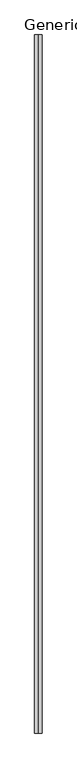
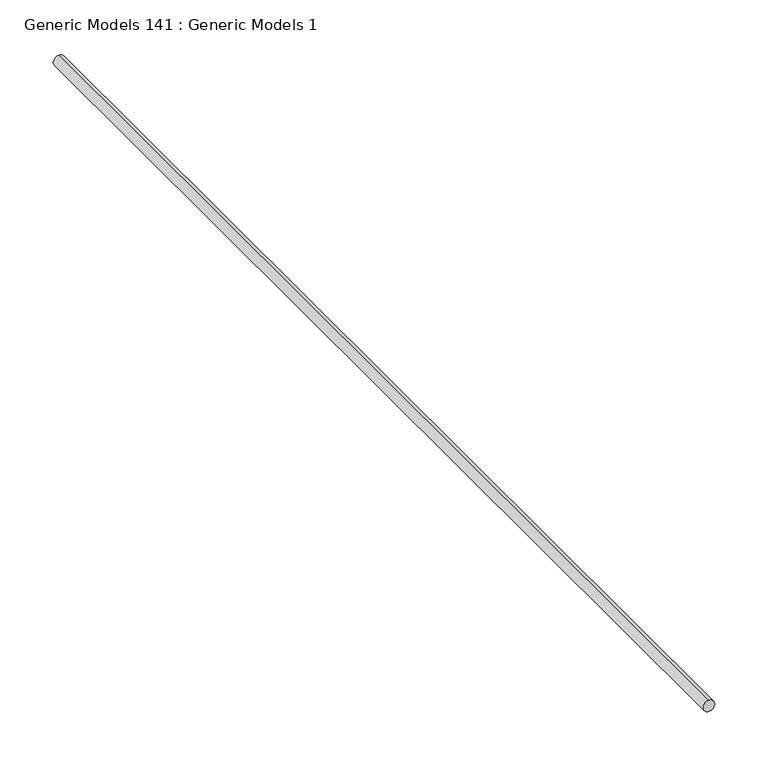
"""IFC4 building model written with IfcOpenShell, lengths in millimetres: proxy geometry, Generic Models 141 : Generic Models 1."""

import ifcopenshell
import ifcopenshell.guid

model = None  # the IFC model being written
_history = None  # IfcOwnerHistory: only IFC2X3 demands one
_inside = {}  # id of a spatial element -> (the spatial element, [elements in it])
_under = {}  # id of a project, library or spatial element -> (it, [spatial elements below it])
_declared = {}  # id of a project -> (the project, [libraries it declares])
_typed = {}  # id of a type object -> (the type object, [elements of that type])
_made_of = {}  # id of a material, layer set ... -> (it, [elements and type objects made of it])


def new_model(schema):
    """Start an empty IFC model of exactly this schema.

    Asked for "IFC4X3", IfcOpenShell would pick the latest addendum, in which some entities
    have other attributes; the version numbers below select the first issue.
    IFC2X3 requires an IfcOwnerHistory on every rooted entity: one is made here for all.
    """
    global model, _history
    if schema == "IFC4X3":
        model = ifcopenshell.file(schema_version=(4, 3, 0, 0))
    else:
        model = ifcopenshell.file(schema=schema)
    _inside.clear()
    _under.clear()
    _declared.clear()
    _typed.clear()
    _made_of.clear()
    _history = None
    if model.schema == "IFC2X3":
        org = make("IfcOrganization", Name="unknown")
        user = make(
            "IfcPersonAndOrganization",
            ThePerson=make("IfcPerson", FamilyName="unknown"),
            TheOrganization=org,
        )
        app = make(
            "IfcApplication",
            ApplicationDeveloper=org,
            Version="unknown",
            ApplicationFullName="unknown",
            ApplicationIdentifier="unknown",
        )
        _history = make(
            "IfcOwnerHistory",
            OwningUser=user,
            OwningApplication=app,
            ChangeAction="ADDED",
            CreationDate=0,
        )
    return model


def make(cls, **values):
    """One entity of the class cls with the attributes given. An attribute that is None is left unset."""
    return model.create_entity(
        cls, **{name: value for name, value in values.items() if value is not None}
    )


def rooted(cls, **values):
    """An entity with a GlobalId (a new one), such as an element, a storey or a relation."""
    return make(cls, GlobalId=ifcopenshell.guid.new(), OwnerHistory=_history, **values)


def si_unit(unit_type, name, prefix=None):
    """IfcSIUnit, for example si_unit("LENGTHUNIT", "METRE", prefix="MILLI")."""
    return make("IfcSIUnit", UnitType=unit_type, Prefix=prefix, Name=name)


def assignment(units):
    """IfcUnitAssignment: the units of a project."""
    return None if units is None else make("IfcUnitAssignment", Units=units)


def point(xyz):
    """IfcCartesianPoint."""
    return None if xyz is None else make("IfcCartesianPoint", Coordinates=xyz)


def direction(xyz):
    """IfcDirection."""
    return None if xyz is None else make("IfcDirection", DirectionRatios=xyz)


def frame(location, z_axis=None, x_axis=None):
    """IfcAxis2Placement3D, a coordinate frame: its origin and axes. An axis left out is left unset."""
    return make(
        "IfcAxis2Placement3D",
        Location=point(location),
        Axis=direction(z_axis),
        RefDirection=direction(x_axis),
    )


def frame_2d(location, x_axis=None):
    """IfcAxis2Placement2D, a coordinate frame in the plane: its origin and x axis."""
    return make(
        "IfcAxis2Placement2D", Location=point(location), RefDirection=direction(x_axis)
    )


def origin():
    """The frame at (0, 0, 0) with its axes left unset."""
    return frame((0.0, 0.0, 0.0))


def place(relative_to, where):
    """IfcLocalPlacement: puts the frame where relative to a parent placement (None: the world)."""
    return make(
        "IfcLocalPlacement", PlacementRelTo=relative_to, RelativePlacement=where
    )


def context(
    kind, dimensions, precision=None, world=None, true_north=None, identifier=None
):
    """IfcGeometricRepresentationContext, for example the 3D "Model" context."""
    return make(
        "IfcGeometricRepresentationContext",
        ContextIdentifier=identifier,
        ContextType=kind,
        CoordinateSpaceDimension=dimensions,
        Precision=precision,
        WorldCoordinateSystem=world,
        TrueNorth=true_north,
    )


def project(units=None, contexts=None):
    """IfcProject with its units and contexts."""
    return rooted(
        "IfcProject",
        Name="project",
        RepresentationContexts=contexts,
        UnitsInContext=assignment(units),
    )


def spatial(cls, under=None, at=None, **own):
    """A site, building, storey or space (cls), placed at a placement, below another one or the project."""
    s = rooted(cls, ObjectPlacement=at, **own)
    if under is not None:
        _under.setdefault(under.id(), (under, []))[1].append(s)
    return s


def circle_curve(where, radius):
    """IfcCircle in the frame where."""
    return make("IfcCircle", Position=where, Radius=radius)


def trimmed(basis, trim1, trim2, sense, master):
    """IfcTrimmedCurve: the piece of a basis curve between two trims."""
    return make(
        "IfcTrimmedCurve",
        BasisCurve=basis,
        Trim1=trim1,
        Trim2=trim2,
        SenseAgreement=sense,
        MasterRepresentation=master,
    )


def segment(curve, same_sense, transition):
    """IfcCompositeCurveSegment."""
    return make(
        "IfcCompositeCurveSegment",
        Transition=transition,
        SameSense=same_sense,
        ParentCurve=curve,
    )


def composite_curve(segments, self_intersect=None):
    """IfcCompositeCurve: segments joined end to end."""
    return make("IfcCompositeCurve", Segments=segments, SelfIntersect=self_intersect)


def outline(outer, holes=None, kind="AREA"):
    """IfcArbitraryClosedProfileDef: a profile drawn as a closed curve; with holes, ...WithVoids."""
    if holes is None:
        return make("IfcArbitraryClosedProfileDef", ProfileType=kind, OuterCurve=outer)
    return make(
        "IfcArbitraryProfileDefWithVoids",
        ProfileType=kind,
        OuterCurve=outer,
        InnerCurves=holes,
    )


def extrude(swept, where, along, depth):
    """IfcExtrudedAreaSolid: the profile swept, set in the frame where, extruded along a direction by depth."""
    return make(
        "IfcExtrudedAreaSolid",
        SweptArea=swept,
        Position=where,
        ExtrudedDirection=direction(along),
        Depth=depth,
    )


def shape(context_of_items, identifier, shape_type, items):
    """IfcShapeRepresentation: the items that make up one representation, for example the "Body"."""
    return make(
        "IfcShapeRepresentation",
        ContextOfItems=context_of_items,
        RepresentationIdentifier=identifier,
        RepresentationType=shape_type,
        Items=items,
    )


def source(mapping_origin, context_of_items, identifier, shape_type, items):
    """IfcRepresentationMap: a shape defined once, which mapped items show again and again."""
    return make(
        "IfcRepresentationMap",
        MappingOrigin=mapping_origin,
        MappedRepresentation=shape(context_of_items, identifier, shape_type, items),
    )


def transform(
    local_origin,
    x_axis=None,
    y_axis=None,
    z_axis=None,
    scale=None,
    scale2=None,
    scale3=None,
    uniform=True,
):
    """IfcCartesianTransformationOperator3D, or its non-uniform kind. x_axis, y_axis, z_axis: its Axis1, 2, 3."""
    if uniform:
        return make(
            "IfcCartesianTransformationOperator3D",
            Axis1=direction(x_axis),
            Axis2=direction(y_axis),
            LocalOrigin=point(local_origin),
            Scale=scale,
            Axis3=direction(z_axis),
        )
    return make(
        "IfcCartesianTransformationOperator3DnonUniform",
        Axis1=direction(x_axis),
        Axis2=direction(y_axis),
        LocalOrigin=point(local_origin),
        Scale=scale,
        Axis3=direction(z_axis),
        Scale2=scale2,
        Scale3=scale3,
    )


def mapped(mapping_source, mapping_target):
    """IfcMappedItem: shows the shape of a source again, moved by a transform."""
    return make(
        "IfcMappedItem", MappingSource=mapping_source, MappingTarget=mapping_target
    )


def made_of(thing, what):
    """Note that an element or type object is made of a material, layer set ...; save() writes the relation."""
    if what is not None:
        _made_of.setdefault(what.id(), (what, []))[1].append(thing)
    return thing


def element(
    cls,
    number,
    at=None,
    inside=None,
    cuts=None,
    type_object=None,
    material=None,
    context=None,
    identifier="Body",
    shape_type=None,
    held_by="IfcProductDefinitionShape",
    body=None,
    shapes=None,
    **own,
):
    """One element of the class cls, such as IfcWall. Its Tag is "e" and its number.

    at: its placement. inside: the storey or other place that contains it. cuts: it is an
    opening in that element (IfcRelVoidsElement). A single representation is given by context,
    identifier, shape_type and body (its items); several are given by shapes. held_by: the class
    of the entity that holds the representations. save() writes the other relations.
    """
    e = rooted(cls, Tag="e%d" % number, ObjectPlacement=at, **own)
    if body is not None:
        shapes = [shape(context, identifier, shape_type, body)]
    if shapes is not None:
        e.Representation = make(held_by, Representations=shapes)
    if inside is not None:
        _inside.setdefault(inside.id(), (inside, []))[1].append(e)
    if cuts is not None:
        rooted(
            "IfcRelVoidsElement", RelatingBuildingElement=cuts, RelatedOpeningElement=e
        )
    if type_object is not None:
        _typed.setdefault(type_object.id(), (type_object, []))[1].append(e)
    return made_of(e, material)


def aggregate(whole, parts):
    """IfcRelAggregates: a whole, such as a stair, and the parts it consists of."""
    return rooted("IfcRelAggregates", RelatingObject=whole, RelatedObjects=parts)


def save(model, path):
    """Write the relations noted so far, then the file.

    IfcRelAggregates (storeys below a building ...), IfcRelContainedInSpatialStructure (elements
    in a storey), IfcRelDefinesByType, IfcRelAssociatesMaterial and IfcRelDeclares: one each for
    every whole, place, type object, material and project.
    """
    for whole, parts in _under.values():
        aggregate(whole, parts)
    for where, things in _inside.values():
        rooted(
            "IfcRelContainedInSpatialStructure",
            RelatedElements=things,
            RelatingStructure=where,
        )
    for kind, things in _typed.values():
        rooted("IfcRelDefinesByType", RelatedObjects=things, RelatingType=kind)
    for what, things in _made_of.values():
        rooted("IfcRelAssociatesMaterial", RelatedObjects=things, RelatingMaterial=what)
    for by, libraries in _declared.values():
        rooted("IfcRelDeclares", RelatingContext=by, RelatedDefinitions=libraries)
    model.write(path)


def generic_models_141_generic_models_1_a1e14504(model_context):
    return source(origin(), model_context, "Body", "SweptSolid", [
        extrude(outline(composite_curve([segment(trimmed(circle_curve(frame_2d((-554.7288266, 52112.9548165)), 6.35), [point((-548.3788266, 52112.9548165))], [point((-561.0788266, 52112.9548165))], False, "CARTESIAN"), True, "CONTINUOUS"), segment(trimmed(circle_curve(frame_2d((-554.7288266, 52112.9548165)), 6.35), [point((-561.0788266, 52112.9548165))], [point((-548.3788266, 52112.9548165))], False, "CARTESIAN"), True, "CONTINUOUS")], self_intersect=False)), frame((0.0, 0.0, 0.0), z_axis=(0.0, 1.0, 0.0), x_axis=(0.0, 0.0, 1.0)), (0.0, 0.0, 1.0), 1219.2),
    ])


if __name__ == "__main__":
    model = new_model("IFC4")
    model_context = context("Model", 3, world=origin())
    ifc_project = project(units=[si_unit("LENGTHUNIT", "METRE", prefix="MILLI")], contexts=[model_context])
    site = spatial("IfcSite", under=ifc_project)
    building = spatial("IfcBuilding", under=site)
    placement = place(None, origin())
    generic_models_141_generic_models_1_shape = generic_models_141_generic_models_1_a1e14504(model_context)
    element("IfcBuildingElementProxy", 1, Name="Generic Models 141 : Generic Models 1", ObjectType="Generic Models 141 : Generic Models 1", at=placement, inside=building, context=model_context, shape_type="MappedRepresentation", body=[
        mapped(generic_models_141_generic_models_1_shape, transform((0.0, 0.0, 0.0), x_axis=(1.0, 0.0, 0.0), y_axis=(0.0, 1.0, 0.0), z_axis=(0.0, 0.0, 1.0))),
    ])
    save(model, "model.ifc")

# Revit data of these elements
# Element 1 (IfcBuildingElementProxy, "Generic Models 141 : Generic Models 1")
#   Materials on its faces: "#4 CONT. STEEL REBAR"
# Materials
#   "#4 CONT. STEEL REBAR": class "Metal", colour RGB 189 187 185, transparency 0, Description = "Structural steel 50ksi", Cost = 0
